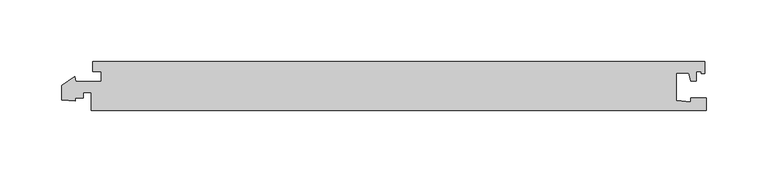
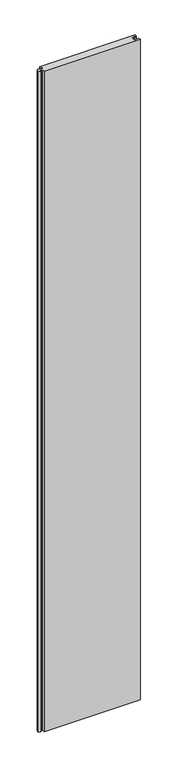
"""IFC4 building model written with IfcOpenShell, lengths in millimetres: proxy geometry, Generic Models 5:Generic Models 5:321804:Generic Models 5:321804 : Generic Models 5:Generic Models 5:321804:25 : Generic Models 5:Generic Models 5:321804:Generic Models 5:321804 : Generic Models 5:Generic Models 5:321804:300761."""

from ifc_helpers import new_model, si_unit, frame, origin, place, context, project, spatial, polyline, outline, extrude, source, transform, mapped, element, save


def generic_models_34c63669(model_context):
    return source(origin(), model_context, "Body", "SweptSolid", [
        extrude(outline(polyline([(583220.2261126, -579052.1037319), (583209.8677824, -579052.1037319), (583209.8677824, -579074.5995222), (583221.8677824, -579075.6493861), (583221.8677824, -579072.4037319), (583234.6177824, -579072.4037319), (583234.6177824, -579082.6037319), (582734.6177824, -579082.6037319), (582734.6177824, -579068.1037319), (582727.9927824, -579068.1037319), (582727.9927824, -579072.4037319), (582721.3677824, -579072.4037319), (582721.3677824, -579075.1037319), (582710.3677824, -579074.1413566), (582710.3677824, -579062.2832156), (582721.0492843, -579055.1758504), (582722.101757, -579059.1037319), (582742.8177824, -579059.1037319), (582742.8177824, -579051.1037319), (582735.8677824, -579051.1037319), (582735.8677824, -579042.6037319), (583233.3677824, -579042.6037319), (583233.3677824, -579052.6037319), (583230.3677824, -579052.6037319), (583230.3677824, -579051.1037319), (583226.4177824, -579051.1037319), (583226.4177824, -579058.6037319), (583221.9677824, -579058.6037319), (583220.2261126, -579052.1037319)])), frame((0.0, 0.0, 30.0324973), z_axis=(0.0, 0.0, 1.0), x_axis=(1.0, 0.0, 0.0)), (0.0, 0.0, 1.0), 3634.8310765),
    ])


if __name__ == "__main__":
    model = new_model("IFC4")
    model_context = context("Model", 3, world=origin())
    ifc_project = project(units=[si_unit("LENGTHUNIT", "METRE", prefix="MILLI")], contexts=[model_context])
    site = spatial("IfcSite", under=ifc_project)
    building = spatial("IfcBuilding", under=site)
    placement = place(None, origin())
    generic_models_shape = generic_models_34c63669(model_context)
    element("IfcBuildingElementProxy", 1, Name="Generic Models 5:Generic Models 5:321804:Generic Models 5:321804 : Generic Models 5:Generic Models 5:321804:25 : Generic Models 5:Generic Models 5:321804:Generic Models 5:321804 : Generic Models 5:Generic Models 5:321804:300761", ObjectType="Generic Models 5:Generic Models 5:321804:Generic Models 5:321804 : Generic Models 5:Generic Models 5:321804:25 : Generic Models 5:Generic Models 5:321804:Generic Models 5:321804 : Generic Models 5:Generic Models 5:321804:300761", at=placement, inside=building, context=model_context, shape_type="MappedRepresentation", body=[
        mapped(generic_models_shape, transform((0.0, 0.0, 0.0), x_axis=(1.0, 0.0, 0.0), y_axis=(0.0, 1.0, 0.0), z_axis=(0.0, 0.0, 1.0))),
    ])
    save(model, "model.ifc")

# Revit data of these elements
# Type "Generic Models 5:Generic Models 5:321804:Generic Models 5:321804 : Generic Models 5:Generic Models 5:321804:25 : Generic Models 5:Generic Models 5:321804:Generic Models 5:321804 : Generic Models 5:Generic Models 5:321804:300761"
#   NameOverride = "Generic Models 5:Generic Models 5:321804:Generic Models 5:321804 : Generic Models 5:Generic Models 5:321804:300761"
#   ObjectTypeOverride = "Generic Models 5:321804 : Generic Models 5:Generic Models 5:321804"
#   Reference = "Generic Models 5"
#   Tag = "300761"
# Element 1 (IfcBuildingElementProxy, "Generic Models 5:Generic Models 5:321804:Generic Models 5:321804 : Generic Models 5:Generic Models 5:321804:25 : Generic Models 5:Generic Models 5:321804:Generic Models 5:321804 : Generic Models 5:Generic Models 5:321804:300761")
#   Materials on its faces: "POLYCARBONATE PANEL - ARCOPLUS 547"
# Materials
#   "POLYCARBONATE PANEL - ARCOPLUS 547": class "Unassigned", colour RGB 202 225 249, transparency 0.45, Cost = 0
